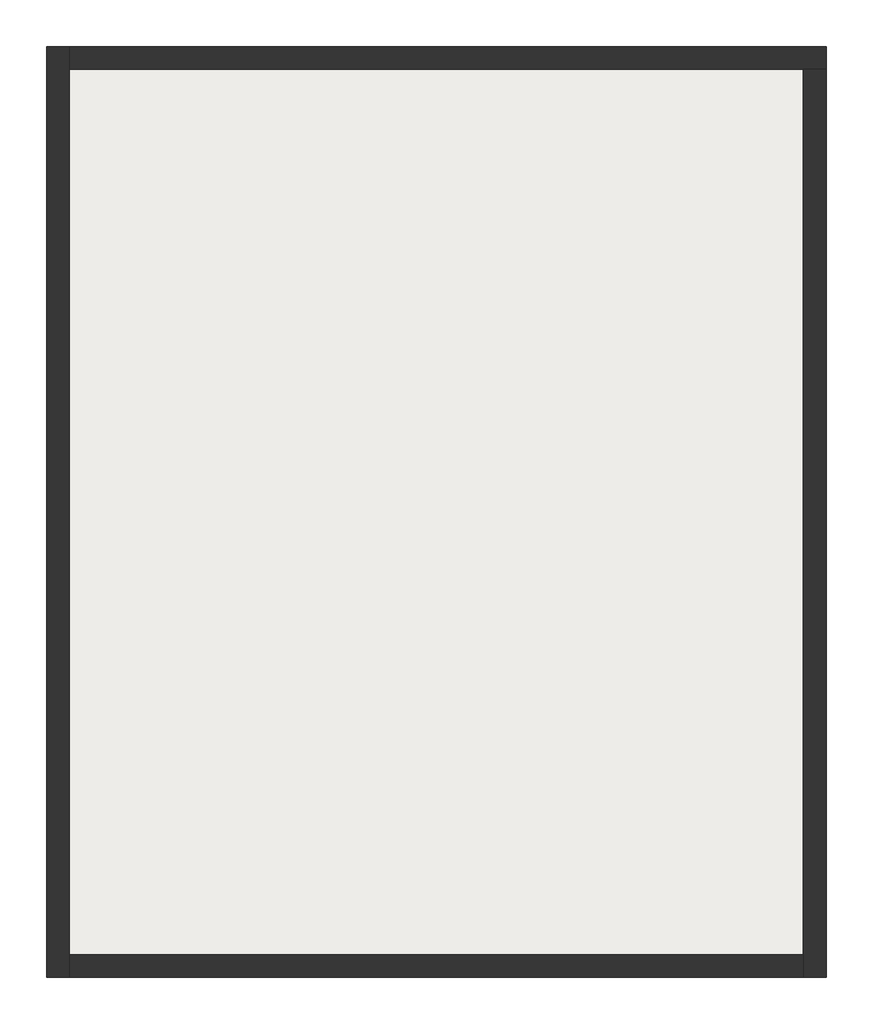
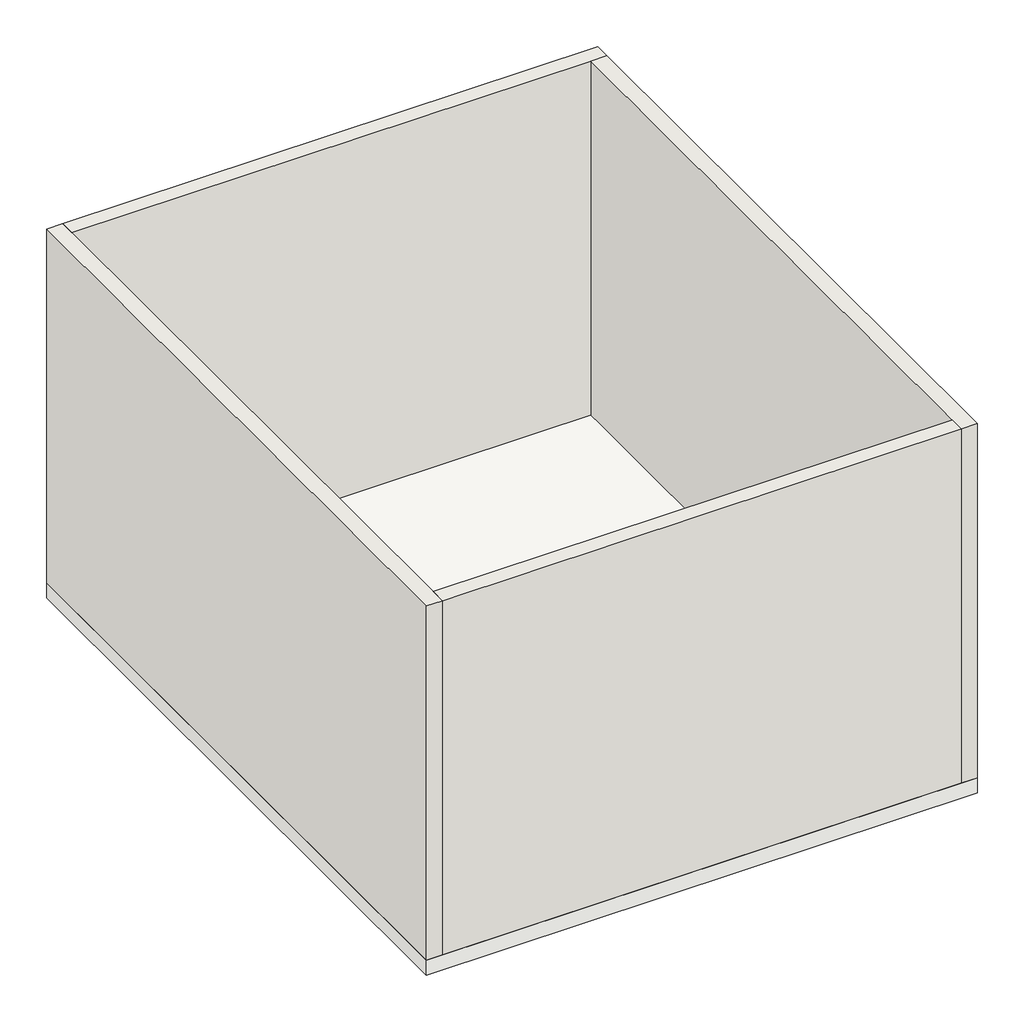
# One storey: 4 walls, 1 slab.
"""IFC4 building model written with IfcOpenShell, lengths in millimetres."""

from ifc_helpers import new_model, si_unit, frame, origin, place, context, project, spatial, polyline, outline, extrude, faceted_brep, element, save

model = new_model("IFC4")

# Units and contexts
model_context = context("Model", 3, world=origin())
ifc_project = project(units=[si_unit("LENGTHUNIT", "METRE", prefix="MILLI")], contexts=[model_context])

# Site, building, storey
site = spatial("IfcSite", under=ifc_project)
building = spatial("IfcBuilding", under=site)
storey = spatial("IfcBuildingStorey", under=building, Name="レベル 1", Elevation=500.0)

# Slab
placement = place(None, origin())
element("IfcSlab", 1, ObjectType="一般 150 mm", at=placement, inside=storey, context=model_context, shape_type="SweptSolid", body=[
    extrude(outline(polyline([(-815.0644277, -1421.7228111), (4334.9355723, -1421.7228111), (4334.9355723, -7571.7228111), (-815.0644277, -7571.7228111), (-815.0644277, -1421.7228111)])), frame((0.0, 0.0, 350.0), z_axis=(0.0, 0.0, 1.0), x_axis=(1.0, 0.0, 0.0)), (0.0, 0.0, 1.0), 150.0),
])

# Walls
element("IfcWall", 2, ObjectType="標準-150mm", at=placement, inside=storey, context=model_context, shape_type="Brep", body=[
    faceted_brep([(-665.0644277, -7571.7228111, 500.0), (-665.0644277, -7421.7228111, 500.0), (-665.0644277, -1571.7228111, 500.0), (-665.0644277, -1421.7228111, 500.0), (-665.0644277, -1421.7228111, 4000.0), (-665.0644277, -1571.7228111, 4000.0), (-665.0644277, -7421.7228111, 4000.0), (-665.0644277, -7571.7228111, 4000.0), (-815.0644277, -7571.7228111, 500.0), (-815.0644277, -7571.7228111, 4000.0), (-815.0644277, -1421.7228111, 4000.0), (-815.0644277, -1421.7228111, 500.0)], [[[0, 1, 2, 3, 4, 5, 6, 7]], [[8, 9, 10, 11]], [[3, 2, 1, 0, 8, 11]], [[7, 6, 5, 4, 10, 9]], [[4, 3, 11, 10]], [[0, 7, 9, 8]]]),
])
element("IfcWall", 3, ObjectType="標準-150mm", at=placement, inside=storey, context=model_context, shape_type="Brep", body=[
    faceted_brep([(-665.0644277, -1571.7228111, 500.0), (4184.9355723, -1571.7228111, 500.0), (4334.9355723, -1571.7228111, 500.0), (4334.9355723, -1571.7228111, 4000.0), (4184.9355723, -1571.7228111, 4000.0), (-665.0644277, -1571.7228111, 4000.0), (-665.0644277, -1421.7228111, 500.0), (-665.0644277, -1421.7228111, 4000.0), (4334.9355723, -1421.7228111, 4000.0), (4334.9355723, -1421.7228111, 500.0)], [[[0, 1, 2, 3, 4, 5]], [[6, 7, 8, 9]], [[2, 1, 0, 6, 9]], [[5, 4, 3, 8, 7]], [[0, 5, 7, 6]], [[3, 2, 9, 8]]]),
])
element("IfcWall", 4, ObjectType="標準-150mm", at=placement, inside=storey, context=model_context, shape_type="Brep", body=[
    faceted_brep([(4184.9355723, -1571.7228111, 500.0), (4184.9355723, -7421.7228111, 500.0), (4184.9355723, -7571.7228111, 500.0), (4184.9355723, -7571.7228111, 4000.0), (4184.9355723, -7421.7228111, 4000.0), (4184.9355723, -1571.7228111, 4000.0), (4334.9355723, -1571.7228111, 500.0), (4334.9355723, -1571.7228111, 4000.0), (4334.9355723, -7571.7228111, 4000.0), (4334.9355723, -7571.7228111, 500.0)], [[[0, 1, 2, 3, 4, 5]], [[6, 7, 8, 9]], [[2, 1, 0, 6, 9]], [[5, 4, 3, 8, 7]], [[0, 5, 7, 6]], [[3, 2, 9, 8]]]),
])
element("IfcWall", 5, ObjectType="標準-150mm", at=placement, inside=storey, context=model_context, shape_type="SweptSolid", body=[
    extrude(outline(polyline([(-665.0644277, -7421.7228111), (4184.9355723, -7421.7228111), (4184.9355723, -7571.7228111), (-665.0644277, -7571.7228111), (-665.0644277, -7421.7228111)])), frame((0.0, 0.0, 500.0), z_axis=(0.0, 0.0, 1.0), x_axis=(1.0, 0.0, 0.0)), (0.0, 0.0, 1.0), 3500.0),
])

save(model, "model.ifc")

# Revit data of these elements
# Project information
#   プロジェクト発行日 = "発行日"
#   プロジェクト ステータス = "プロジェクト ステータス"
#   クライアント名 = "オーナ"
#   計画地住所 = "ここにアドレスを入力"
#   プロジェクト名 = "プロジェクト名"
#   プロジェクト番号 = "0001"
# Type "一般 150 mm"
#   Function = 0
#   Layers, outside or top first: 150 mm no material (function 1)
# Type "標準-150mm"
#   Layers, outside or top first: 150 mm no material (function 1)
# Element 1 (IfcSlab, "一般 150 mm")
#   built-in parameter 1001955 = 1.5708 (stored number, unit not read)
#   Height Offset From Level = 0 mm
#   Phase Created = 新しい建設
# Elements 2, 3, 4, 5 (IfcWall, "標準-150mm")
#   Top Offset = 0 mm
#   Base Offset = 0 mm
#   wall height = 3500 mm
#   Phase Created = 新しい建設
#   Base Constraint = レベル 1
#   Top Constraint = レベル 2
#   Materials on its faces: "既定の壁"
# Materials
#   "既定の壁": class "その他", colour RGB 127 127 127, transparency 0, Cost = 0
# Room, not placed, phase "新しい建設", upper offset 0 mm, lower offset 0 mm
#   Number = "1"
#   Name = "部屋"
# Room, not placed, phase "新しい建設", upper offset 0 mm, lower offset 0 mm
#   Number = "2"
#   Name = "部屋"
# Room, not placed, phase "新しい建設", upper offset 0 mm, lower offset 0 mm
#   Number = "3"
#   Name = "部屋"
# Room at (1693.246, -4711.323) mm, phase "新しい建設", upper level "レベル 1", upper offset 3500 mm, lower offset 0 mm
#   Number = "4"
#   Name = "部屋"
